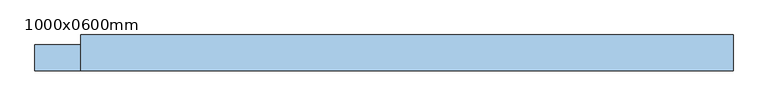
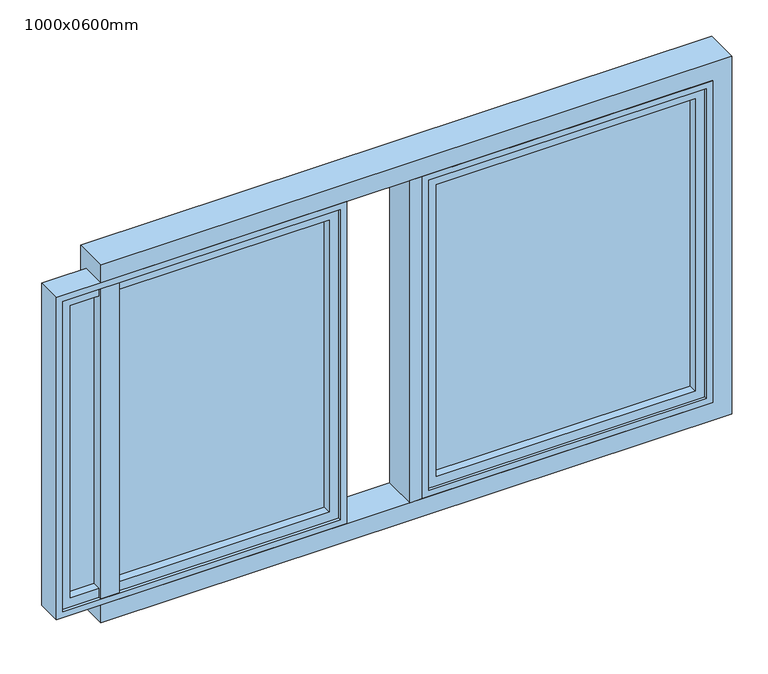
"""IFC4 building model written with IfcOpenShell, lengths in millimetres: window geometry, Janela Maxim-air - 2 Módulos : 1000x0600mm."""

import ifcopenshell
import ifcopenshell.guid

model = None  # the IFC model being written
_history = None  # IfcOwnerHistory: only IFC2X3 demands one
_inside = {}  # id of a spatial element -> (the spatial element, [elements in it])
_under = {}  # id of a project, library or spatial element -> (it, [spatial elements below it])
_declared = {}  # id of a project -> (the project, [libraries it declares])
_typed = {}  # id of a type object -> (the type object, [elements of that type])
_made_of = {}  # id of a material, layer set ... -> (it, [elements and type objects made of it])


def new_model(schema):
    """Start an empty IFC model of exactly this schema.

    Asked for "IFC4X3", IfcOpenShell would pick the latest addendum, in which some entities
    have other attributes; the version numbers below select the first issue.
    IFC2X3 requires an IfcOwnerHistory on every rooted entity: one is made here for all.
    """
    global model, _history
    if schema == "IFC4X3":
        model = ifcopenshell.file(schema_version=(4, 3, 0, 0))
    else:
        model = ifcopenshell.file(schema=schema)
    _inside.clear()
    _under.clear()
    _declared.clear()
    _typed.clear()
    _made_of.clear()
    _history = None
    if model.schema == "IFC2X3":
        org = make("IfcOrganization", Name="unknown")
        user = make(
            "IfcPersonAndOrganization",
            ThePerson=make("IfcPerson", FamilyName="unknown"),
            TheOrganization=org,
        )
        app = make(
            "IfcApplication",
            ApplicationDeveloper=org,
            Version="unknown",
            ApplicationFullName="unknown",
            ApplicationIdentifier="unknown",
        )
        _history = make(
            "IfcOwnerHistory",
            OwningUser=user,
            OwningApplication=app,
            ChangeAction="ADDED",
            CreationDate=0,
        )
    return model


def make(cls, **values):
    """One entity of the class cls with the attributes given. An attribute that is None is left unset."""
    return model.create_entity(
        cls, **{name: value for name, value in values.items() if value is not None}
    )


def rooted(cls, **values):
    """An entity with a GlobalId (a new one), such as an element, a storey or a relation."""
    return make(cls, GlobalId=ifcopenshell.guid.new(), OwnerHistory=_history, **values)


def si_unit(unit_type, name, prefix=None):
    """IfcSIUnit, for example si_unit("LENGTHUNIT", "METRE", prefix="MILLI")."""
    return make("IfcSIUnit", UnitType=unit_type, Prefix=prefix, Name=name)


def assignment(units):
    """IfcUnitAssignment: the units of a project."""
    return None if units is None else make("IfcUnitAssignment", Units=units)


def point(xyz):
    """IfcCartesianPoint."""
    return None if xyz is None else make("IfcCartesianPoint", Coordinates=xyz)


def direction(xyz):
    """IfcDirection."""
    return None if xyz is None else make("IfcDirection", DirectionRatios=xyz)


def frame(location, z_axis=None, x_axis=None):
    """IfcAxis2Placement3D, a coordinate frame: its origin and axes. An axis left out is left unset."""
    return make(
        "IfcAxis2Placement3D",
        Location=point(location),
        Axis=direction(z_axis),
        RefDirection=direction(x_axis),
    )


def origin():
    """The frame at (0, 0, 0) with its axes left unset."""
    return frame((0.0, 0.0, 0.0))


def place(relative_to, where):
    """IfcLocalPlacement: puts the frame where relative to a parent placement (None: the world)."""
    return make(
        "IfcLocalPlacement", PlacementRelTo=relative_to, RelativePlacement=where
    )


def context(
    kind, dimensions, precision=None, world=None, true_north=None, identifier=None
):
    """IfcGeometricRepresentationContext, for example the 3D "Model" context."""
    return make(
        "IfcGeometricRepresentationContext",
        ContextIdentifier=identifier,
        ContextType=kind,
        CoordinateSpaceDimension=dimensions,
        Precision=precision,
        WorldCoordinateSystem=world,
        TrueNorth=true_north,
    )


def project(units=None, contexts=None):
    """IfcProject with its units and contexts."""
    return rooted(
        "IfcProject",
        Name="project",
        RepresentationContexts=contexts,
        UnitsInContext=assignment(units),
    )


def spatial(cls, under=None, at=None, **own):
    """A site, building, storey or space (cls), placed at a placement, below another one or the project."""
    s = rooted(cls, ObjectPlacement=at, **own)
    if under is not None:
        _under.setdefault(under.id(), (under, []))[1].append(s)
    return s


def polyline(points):
    """IfcPolyline through the points."""
    return make("IfcPolyline", Points=[point(p) for p in points])


def outline(outer, holes=None, kind="AREA"):
    """IfcArbitraryClosedProfileDef: a profile drawn as a closed curve; with holes, ...WithVoids."""
    if holes is None:
        return make("IfcArbitraryClosedProfileDef", ProfileType=kind, OuterCurve=outer)
    return make(
        "IfcArbitraryProfileDefWithVoids",
        ProfileType=kind,
        OuterCurve=outer,
        InnerCurves=holes,
    )


def extrude(swept, where, along, depth):
    """IfcExtrudedAreaSolid: the profile swept, set in the frame where, extruded along a direction by depth."""
    return make(
        "IfcExtrudedAreaSolid",
        SweptArea=swept,
        Position=where,
        ExtrudedDirection=direction(along),
        Depth=depth,
    )


def faces_of(points, faces, orient=None, outer=None):
    """IfcFace entities. A face is a list of loops; a loop is a list of indices into points, from 0.

    orient and outer hold one flag for each loop. By default every Orientation is true, the
    first loop of a face is its IfcFaceOuterBound and the others are IfcFaceBound.
    """
    made = []
    for i, loops in enumerate(faces):
        bounds = []
        for j, loop in enumerate(loops):
            is_outer = j == 0 if outer is None else outer[i][j]
            bounds.append(
                make(
                    "IfcFaceOuterBound" if is_outer else "IfcFaceBound",
                    Bound=make("IfcPolyLoop", Polygon=[points[k] for k in loop]),
                    Orientation=True if orient is None else orient[i][j],
                )
            )
        made.append(make("IfcFace", Bounds=bounds))
    return made


def faceted_brep(points, faces, orient=None, outer=None, voids=None):
    """IfcFacetedBrep: a solid bounded by flat faces; with voids (closed shells), ...WithVoids."""
    shared = [point(p) for p in points]
    hull = make("IfcClosedShell", CfsFaces=faces_of(shared, faces, orient, outer))
    if voids is None:
        return make("IfcFacetedBrep", Outer=hull)
    return make(
        "IfcFacetedBrepWithVoids",
        Outer=hull,
        Voids=[
            make(cls, CfsFaces=faces_of(shared, fs, o, b)) for cls, fs, o, b in voids
        ],
    )


def shape(context_of_items, identifier, shape_type, items):
    """IfcShapeRepresentation: the items that make up one representation, for example the "Body"."""
    return make(
        "IfcShapeRepresentation",
        ContextOfItems=context_of_items,
        RepresentationIdentifier=identifier,
        RepresentationType=shape_type,
        Items=items,
    )


def source(mapping_origin, context_of_items, identifier, shape_type, items):
    """IfcRepresentationMap: a shape defined once, which mapped items show again and again."""
    return make(
        "IfcRepresentationMap",
        MappingOrigin=mapping_origin,
        MappedRepresentation=shape(context_of_items, identifier, shape_type, items),
    )


def transform(
    local_origin,
    x_axis=None,
    y_axis=None,
    z_axis=None,
    scale=None,
    scale2=None,
    scale3=None,
    uniform=True,
):
    """IfcCartesianTransformationOperator3D, or its non-uniform kind. x_axis, y_axis, z_axis: its Axis1, 2, 3."""
    if uniform:
        return make(
            "IfcCartesianTransformationOperator3D",
            Axis1=direction(x_axis),
            Axis2=direction(y_axis),
            LocalOrigin=point(local_origin),
            Scale=scale,
            Axis3=direction(z_axis),
        )
    return make(
        "IfcCartesianTransformationOperator3DnonUniform",
        Axis1=direction(x_axis),
        Axis2=direction(y_axis),
        LocalOrigin=point(local_origin),
        Scale=scale,
        Axis3=direction(z_axis),
        Scale2=scale2,
        Scale3=scale3,
    )


def mapped(mapping_source, mapping_target):
    """IfcMappedItem: shows the shape of a source again, moved by a transform."""
    return make(
        "IfcMappedItem", MappingSource=mapping_source, MappingTarget=mapping_target
    )


def made_of(thing, what):
    """Note that an element or type object is made of a material, layer set ...; save() writes the relation."""
    if what is not None:
        _made_of.setdefault(what.id(), (what, []))[1].append(thing)
    return thing


def element(
    cls,
    number,
    at=None,
    inside=None,
    cuts=None,
    type_object=None,
    material=None,
    context=None,
    identifier="Body",
    shape_type=None,
    held_by="IfcProductDefinitionShape",
    body=None,
    shapes=None,
    **own,
):
    """One element of the class cls, such as IfcWall. Its Tag is "e" and its number.

    at: its placement. inside: the storey or other place that contains it. cuts: it is an
    opening in that element (IfcRelVoidsElement). A single representation is given by context,
    identifier, shape_type and body (its items); several are given by shapes. held_by: the class
    of the entity that holds the representations. save() writes the other relations.
    """
    e = rooted(cls, Tag="e%d" % number, ObjectPlacement=at, **own)
    if body is not None:
        shapes = [shape(context, identifier, shape_type, body)]
    if shapes is not None:
        e.Representation = make(held_by, Representations=shapes)
    if inside is not None:
        _inside.setdefault(inside.id(), (inside, []))[1].append(e)
    if cuts is not None:
        rooted(
            "IfcRelVoidsElement", RelatingBuildingElement=cuts, RelatedOpeningElement=e
        )
    if type_object is not None:
        _typed.setdefault(type_object.id(), (type_object, []))[1].append(e)
    return made_of(e, material)


def aggregate(whole, parts):
    """IfcRelAggregates: a whole, such as a stair, and the parts it consists of."""
    return rooted("IfcRelAggregates", RelatingObject=whole, RelatedObjects=parts)


def save(model, path):
    """Write the relations noted so far, then the file.

    IfcRelAggregates (storeys below a building ...), IfcRelContainedInSpatialStructure (elements
    in a storey), IfcRelDefinesByType, IfcRelAssociatesMaterial and IfcRelDeclares: one each for
    every whole, place, type object, material and project.
    """
    for whole, parts in _under.values():
        aggregate(whole, parts)
    for where, things in _inside.values():
        rooted(
            "IfcRelContainedInSpatialStructure",
            RelatedElements=things,
            RelatingStructure=where,
        )
    for kind, things in _typed.values():
        rooted("IfcRelDefinesByType", RelatedObjects=things, RelatingType=kind)
    for what, things in _made_of.values():
        rooted("IfcRelAssociatesMaterial", RelatedObjects=things, RelatingMaterial=what)
    for by, libraries in _declared.values():
        rooted("IfcRelDeclares", RelatingContext=by, RelatedDefinitions=libraries)
    model.write(path)


def window_1000x0600mm_9fc04acc(model_context):
    return source(origin(), model_context, "Body", "SolidModel", [
        extrude(outline(polyline([(452.0, 51.3), (28.0, 51.3), (28.0, 58.3), (452.0, 58.3), (452.0, 51.3)])), frame((0.0, 0.0, 1048.0), z_axis=(0.0, 0.0, 1.0), x_axis=(1.0, 0.0, 0.0)), (0.0, 0.0, 1.0), 504.0),
        faceted_brep([(35.0, 72.3, 1545.0), (35.0, 58.3, 1545.0), (35.0, 58.3, 1055.0), (35.0, 72.3, 1055.0), (28.0, 58.3, 1552.0), (28.0, 51.3, 1552.0), (28.0, 51.3, 1048.0), (28.0, 58.3, 1048.0), (35.0, 51.3, 1545.0), (35.0, 37.3, 1545.0), (35.0, 37.3, 1055.0), (35.0, 51.3, 1055.0), (15.0, 37.3, 1565.0), (15.0, 72.3, 1565.0), (15.0, 72.3, 1035.0), (15.0, 37.3, 1035.0), (445.0, 58.3, 1055.0), (445.0, 72.3, 1055.0), (452.0, 51.3, 1048.0), (452.0, 58.3, 1048.0), (445.0, 37.3, 1055.0), (445.0, 51.3, 1055.0), (465.0, 72.3, 1035.0), (465.0, 37.3, 1035.0), (445.0, 58.3, 1545.0), (445.0, 72.3, 1545.0), (452.0, 51.3, 1552.0), (452.0, 58.3, 1552.0), (445.0, 37.3, 1545.0), (445.0, 51.3, 1545.0), (465.0, 72.3, 1565.0), (465.0, 37.3, 1565.0)], [[[0, 1, 2, 3]], [[4, 5, 6, 7]], [[8, 9, 10, 11]], [[12, 13, 14, 15]], [[3, 2, 16, 17]], [[7, 6, 18, 19]], [[11, 10, 20, 21]], [[15, 14, 22, 23]], [[17, 16, 24, 25]], [[19, 18, 26, 27]], [[21, 20, 28, 29]], [[23, 22, 30, 31]], [[13, 30, 22, 14], [3, 17, 25, 0]], [[25, 24, 1, 0]], [[7, 19, 27, 4], [1, 24, 16, 2]], [[27, 26, 5, 4]], [[5, 26, 18, 6], [11, 21, 29, 8]], [[29, 28, 9, 8]], [[15, 23, 31, 12], [9, 28, 20, 10]], [[31, 30, 13, 12]]]),
        faceted_brep([(15.0, 72.3, 1565.0), (15.0, 37.3, 1565.0), (15.0, 37.3, 1035.0), (15.0, 72.3, 1035.0), (20.0, 37.3, 1560.0), (20.0, 32.3, 1560.0), (20.0, 32.3, 1040.0), (20.0, 37.3, 1040.0), (10.0, 32.3, 1570.0), (10.0, 72.3, 1570.0), (10.0, 72.3, 1030.0), (10.0, 32.3, 1030.0), (465.0, 37.3, 1035.0), (465.0, 72.3, 1035.0), (460.0, 32.3, 1040.0), (460.0, 37.3, 1040.0), (470.0, 72.3, 1030.0), (470.0, 32.3, 1030.0), (465.0, 37.3, 1565.0), (465.0, 72.3, 1565.0), (460.0, 32.3, 1560.0), (460.0, 37.3, 1560.0), (470.0, 72.3, 1570.0), (470.0, 32.3, 1570.0)], [[[0, 1, 2, 3]], [[4, 5, 6, 7]], [[8, 9, 10, 11]], [[3, 2, 12, 13]], [[7, 6, 14, 15]], [[11, 10, 16, 17]], [[13, 12, 18, 19]], [[15, 14, 20, 21]], [[17, 16, 22, 23]], [[9, 22, 16, 10], [3, 13, 19, 0]], [[19, 18, 1, 0]], [[1, 18, 12, 2], [7, 15, 21, 4]], [[21, 20, 5, 4]], [[11, 17, 23, 8], [5, 20, 14, 6]], [[23, 22, 9, 8]]]),
        extrude(outline(polyline([(-552.0, 51.3), (-552.0, 58.3), (-128.0, 58.3), (-128.0, 51.3), (-552.0, 51.3)])), frame((0.0, 0.0, 1048.0), z_axis=(0.0, 0.0, 1.0), x_axis=(1.0, 0.0, 0.0)), (0.0, 0.0, 1.0), 504.0),
        faceted_brep([(-135.0, 72.3, 1545.0), (-135.0, 72.3, 1055.0), (-135.0, 58.3, 1055.0), (-135.0, 58.3, 1545.0), (-128.0, 58.3, 1552.0), (-128.0, 58.3, 1048.0), (-128.0, 51.3, 1048.0), (-128.0, 51.3, 1552.0), (-135.0, 51.3, 1545.0), (-135.0, 51.3, 1055.0), (-135.0, 37.3, 1055.0), (-135.0, 37.3, 1545.0), (-115.0, 37.3, 1565.0), (-115.0, 37.3, 1035.0), (-115.0, 72.3, 1035.0), (-115.0, 72.3, 1565.0), (-545.0, 72.3, 1055.0), (-545.0, 58.3, 1055.0), (-552.0, 58.3, 1048.0), (-552.0, 51.3, 1048.0), (-545.0, 51.3, 1055.0), (-545.0, 37.3, 1055.0), (-565.0, 37.3, 1035.0), (-565.0, 72.3, 1035.0), (-545.0, 72.3, 1545.0), (-545.0, 58.3, 1545.0), (-552.0, 58.3, 1552.0), (-552.0, 51.3, 1552.0), (-545.0, 51.3, 1545.0), (-545.0, 37.3, 1545.0), (-565.0, 37.3, 1565.0), (-565.0, 72.3, 1565.0)], [[[0, 1, 2, 3]], [[4, 5, 6, 7]], [[8, 9, 10, 11]], [[12, 13, 14, 15]], [[1, 16, 17, 2]], [[5, 18, 19, 6]], [[9, 20, 21, 10]], [[13, 22, 23, 14]], [[16, 24, 25, 17]], [[18, 26, 27, 19]], [[20, 28, 29, 21]], [[22, 30, 31, 23]], [[15, 14, 23, 31], [1, 0, 24, 16]], [[24, 0, 3, 25]], [[5, 4, 26, 18], [3, 2, 17, 25]], [[26, 4, 7, 27]], [[7, 6, 19, 27], [9, 8, 28, 20]], [[28, 8, 11, 29]], [[13, 12, 30, 22], [11, 10, 21, 29]], [[30, 12, 15, 31]]]),
        faceted_brep([(-115.0, 72.3, 1565.0), (-115.0, 72.3, 1035.0), (-115.0, 37.3, 1035.0), (-115.0, 37.3, 1565.0), (-120.0, 37.3, 1560.0), (-120.0, 37.3, 1040.0), (-120.0, 32.3, 1040.0), (-120.0, 32.3, 1560.0), (-110.0, 32.3, 1570.0), (-110.0, 32.3, 1030.0), (-110.0, 72.3, 1030.0), (-110.0, 72.3, 1570.0), (-565.0, 72.3, 1035.0), (-565.0, 37.3, 1035.0), (-560.0, 37.3, 1040.0), (-560.0, 32.3, 1040.0), (-570.0, 32.3, 1030.0), (-570.0, 72.3, 1030.0), (-565.0, 72.3, 1565.0), (-565.0, 37.3, 1565.0), (-560.0, 37.3, 1560.0), (-560.0, 32.3, 1560.0), (-570.0, 32.3, 1570.0), (-570.0, 72.3, 1570.0)], [[[0, 1, 2, 3]], [[4, 5, 6, 7]], [[8, 9, 10, 11]], [[1, 12, 13, 2]], [[5, 14, 15, 6]], [[9, 16, 17, 10]], [[12, 18, 19, 13]], [[14, 20, 21, 15]], [[16, 22, 23, 17]], [[11, 10, 17, 23], [1, 0, 18, 12]], [[18, 0, 3, 19]], [[3, 2, 13, 19], [5, 4, 20, 14]], [[20, 4, 7, 21]], [[9, 8, 22, 16], [7, 6, 15, 21]], [[22, 8, 11, 23]]]),
        extrude(outline(polyline([(10.0, 87.3), (10.0, 32.3), (-10.0, 32.3), (-10.0, 87.3), (10.0, 87.3)])), frame((0.0, 0.0, 1030.0), z_axis=(0.0, 0.0, 1.0), x_axis=(1.0, 0.0, 0.0)), (0.0, 0.0, 1.0), 540.0),
        extrude(outline(polyline([(1000.0, 500.0), (1600.0, 500.0), (1600.0, -500.0), (1000.0, -500.0), (1000.0, 500.0)]), holes=[polyline([(1570.0, 470.0), (1030.0, 470.0), (1030.0, -470.0), (1570.0, -470.0), (1570.0, 470.0)])]), frame((0.0, 32.3, 0.0), z_axis=(0.0, 1.0, 0.0), x_axis=(0.0, 0.0, 1.0)), (0.0, 0.0, 1.0), 55.0),
    ])


if __name__ == "__main__":
    model = new_model("IFC4")
    model_context = context("Model", 3, world=origin())
    ifc_project = project(units=[si_unit("LENGTHUNIT", "METRE", prefix="MILLI")], contexts=[model_context])
    site = spatial("IfcSite", under=ifc_project)
    building = spatial("IfcBuilding", under=site)
    placement = place(None, origin())
    window_1000x0600mm_shape = window_1000x0600mm_9fc04acc(model_context)
    element("IfcWindow", 1, ObjectType="Janela Maxim-air - 2 Módulos : 1000x0600mm", at=placement, inside=building, context=model_context, shape_type="MappedRepresentation", body=[
        mapped(window_1000x0600mm_shape, transform((0.0, 0.0, 0.0), x_axis=(1.0, 0.0, 0.0), y_axis=(0.0, 1.0, 0.0), z_axis=(0.0, 0.0, 1.0))),
    ])
    save(model, "model.ifc")

# Revit data of these elements
# Type "Janela Maxim-air - 2 Módulos : 1000x0600mm"
#   Type Mark = "J12"
#   SINAPI = ""
#   ref. vert. basc. = 0.54 m
#   ref. horiz. basc. = 0.46 m
#   Largura Batente = 0.055 m
#   Height = 0.60 m
#   Default Sill Height = 1.00 m
#   Width = 1.00 m
#   Material Quadro = Metal - Alumínio
#   Material Painel = Vidro
#   Wall Closure = (empty or 0)
#   Assembly Code = ""
# Element 1 (IfcWindow, "Janela Maxim-air - 2 Módulos : 1000x0600mm")
#   Materials on its faces: "Metal - Alumínio", "Vidro"
# Materials
#   "Metal - Alumínio": class "Metal", colour RGB 244 244 244, transparency 0
#   "Vidro": class "Vidro", colour RGB 0 128 192, transparency 0.9, Description = "Vidro de sílica", Cost = 0
